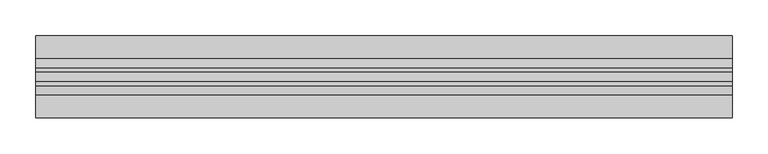
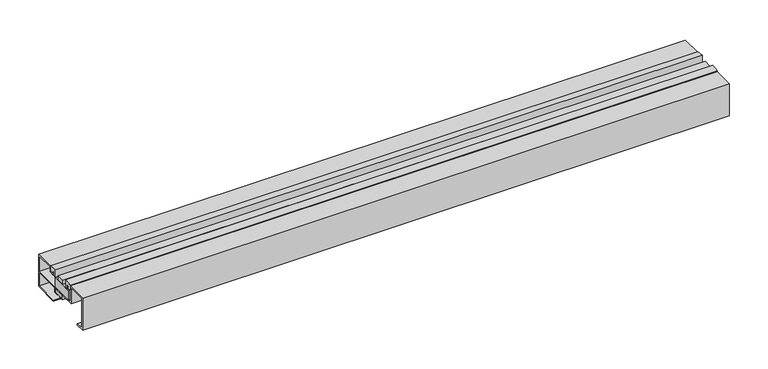
"""IFC4 building model written with IfcOpenShell, lengths in millimetres: proxy geometry, Generic Models 3:Generic Models 1:2:Generic Models 1:2 : Generic Models 3:Generic Models 1:300625:328150:Generic Models 1:2:Generic Models 1:2 : Generic Models 3:Generic Models 1:300625:328150 : Generic Models 3:Generic Models 1:2:Generic Models 1:2 : Generic Models 3:Generic Models 1:300625:328150:1 : Generic Models 3:Generic Models 1:2:Generic Models 1:2 : Generic Models 3:Generic Models 1:300625:328150:Generic Models 1:2:Generic Models 1:2 : Generic Models 3:Generic Models 1:300625:328150 : Generic Models 3:Generic Models 1:2:Generic Models 1:2 : Generic Models 3:Generic Models 1:300625:328150:300962."""

import ifcopenshell
import ifcopenshell.guid

model = None  # the IFC model being written
_history = None  # IfcOwnerHistory: only IFC2X3 demands one
_inside = {}  # id of a spatial element -> (the spatial element, [elements in it])
_under = {}  # id of a project, library or spatial element -> (it, [spatial elements below it])
_declared = {}  # id of a project -> (the project, [libraries it declares])
_typed = {}  # id of a type object -> (the type object, [elements of that type])
_made_of = {}  # id of a material, layer set ... -> (it, [elements and type objects made of it])


def new_model(schema):
    """Start an empty IFC model of exactly this schema.

    Asked for "IFC4X3", IfcOpenShell would pick the latest addendum, in which some entities
    have other attributes; the version numbers below select the first issue.
    IFC2X3 requires an IfcOwnerHistory on every rooted entity: one is made here for all.
    """
    global model, _history
    if schema == "IFC4X3":
        model = ifcopenshell.file(schema_version=(4, 3, 0, 0))
    else:
        model = ifcopenshell.file(schema=schema)
    _inside.clear()
    _under.clear()
    _declared.clear()
    _typed.clear()
    _made_of.clear()
    _history = None
    if model.schema == "IFC2X3":
        org = make("IfcOrganization", Name="unknown")
        user = make(
            "IfcPersonAndOrganization",
            ThePerson=make("IfcPerson", FamilyName="unknown"),
            TheOrganization=org,
        )
        app = make(
            "IfcApplication",
            ApplicationDeveloper=org,
            Version="unknown",
            ApplicationFullName="unknown",
            ApplicationIdentifier="unknown",
        )
        _history = make(
            "IfcOwnerHistory",
            OwningUser=user,
            OwningApplication=app,
            ChangeAction="ADDED",
            CreationDate=0,
        )
    return model


def make(cls, **values):
    """One entity of the class cls with the attributes given. An attribute that is None is left unset."""
    return model.create_entity(
        cls, **{name: value for name, value in values.items() if value is not None}
    )


def rooted(cls, **values):
    """An entity with a GlobalId (a new one), such as an element, a storey or a relation."""
    return make(cls, GlobalId=ifcopenshell.guid.new(), OwnerHistory=_history, **values)


def si_unit(unit_type, name, prefix=None):
    """IfcSIUnit, for example si_unit("LENGTHUNIT", "METRE", prefix="MILLI")."""
    return make("IfcSIUnit", UnitType=unit_type, Prefix=prefix, Name=name)


def assignment(units):
    """IfcUnitAssignment: the units of a project."""
    return None if units is None else make("IfcUnitAssignment", Units=units)


def point(xyz):
    """IfcCartesianPoint."""
    return None if xyz is None else make("IfcCartesianPoint", Coordinates=xyz)


def direction(xyz):
    """IfcDirection."""
    return None if xyz is None else make("IfcDirection", DirectionRatios=xyz)


def frame(location, z_axis=None, x_axis=None):
    """IfcAxis2Placement3D, a coordinate frame: its origin and axes. An axis left out is left unset."""
    return make(
        "IfcAxis2Placement3D",
        Location=point(location),
        Axis=direction(z_axis),
        RefDirection=direction(x_axis),
    )


def origin():
    """The frame at (0, 0, 0) with its axes left unset."""
    return frame((0.0, 0.0, 0.0))


def place(relative_to, where):
    """IfcLocalPlacement: puts the frame where relative to a parent placement (None: the world)."""
    return make(
        "IfcLocalPlacement", PlacementRelTo=relative_to, RelativePlacement=where
    )


def context(
    kind, dimensions, precision=None, world=None, true_north=None, identifier=None
):
    """IfcGeometricRepresentationContext, for example the 3D "Model" context."""
    return make(
        "IfcGeometricRepresentationContext",
        ContextIdentifier=identifier,
        ContextType=kind,
        CoordinateSpaceDimension=dimensions,
        Precision=precision,
        WorldCoordinateSystem=world,
        TrueNorth=true_north,
    )


def project(units=None, contexts=None):
    """IfcProject with its units and contexts."""
    return rooted(
        "IfcProject",
        Name="project",
        RepresentationContexts=contexts,
        UnitsInContext=assignment(units),
    )


def spatial(cls, under=None, at=None, **own):
    """A site, building, storey or space (cls), placed at a placement, below another one or the project."""
    s = rooted(cls, ObjectPlacement=at, **own)
    if under is not None:
        _under.setdefault(under.id(), (under, []))[1].append(s)
    return s


def polyline(points):
    """IfcPolyline through the points."""
    return make("IfcPolyline", Points=[point(p) for p in points])


def outline(outer, holes=None, kind="AREA"):
    """IfcArbitraryClosedProfileDef: a profile drawn as a closed curve; with holes, ...WithVoids."""
    if holes is None:
        return make("IfcArbitraryClosedProfileDef", ProfileType=kind, OuterCurve=outer)
    return make(
        "IfcArbitraryProfileDefWithVoids",
        ProfileType=kind,
        OuterCurve=outer,
        InnerCurves=holes,
    )


def extrude(swept, where, along, depth):
    """IfcExtrudedAreaSolid: the profile swept, set in the frame where, extruded along a direction by depth."""
    return make(
        "IfcExtrudedAreaSolid",
        SweptArea=swept,
        Position=where,
        ExtrudedDirection=direction(along),
        Depth=depth,
    )


def shape(context_of_items, identifier, shape_type, items):
    """IfcShapeRepresentation: the items that make up one representation, for example the "Body"."""
    return make(
        "IfcShapeRepresentation",
        ContextOfItems=context_of_items,
        RepresentationIdentifier=identifier,
        RepresentationType=shape_type,
        Items=items,
    )


def source(mapping_origin, context_of_items, identifier, shape_type, items):
    """IfcRepresentationMap: a shape defined once, which mapped items show again and again."""
    return make(
        "IfcRepresentationMap",
        MappingOrigin=mapping_origin,
        MappedRepresentation=shape(context_of_items, identifier, shape_type, items),
    )


def transform(
    local_origin,
    x_axis=None,
    y_axis=None,
    z_axis=None,
    scale=None,
    scale2=None,
    scale3=None,
    uniform=True,
):
    """IfcCartesianTransformationOperator3D, or its non-uniform kind. x_axis, y_axis, z_axis: its Axis1, 2, 3."""
    if uniform:
        return make(
            "IfcCartesianTransformationOperator3D",
            Axis1=direction(x_axis),
            Axis2=direction(y_axis),
            LocalOrigin=point(local_origin),
            Scale=scale,
            Axis3=direction(z_axis),
        )
    return make(
        "IfcCartesianTransformationOperator3DnonUniform",
        Axis1=direction(x_axis),
        Axis2=direction(y_axis),
        LocalOrigin=point(local_origin),
        Scale=scale,
        Axis3=direction(z_axis),
        Scale2=scale2,
        Scale3=scale3,
    )


def mapped(mapping_source, mapping_target):
    """IfcMappedItem: shows the shape of a source again, moved by a transform."""
    return make(
        "IfcMappedItem", MappingSource=mapping_source, MappingTarget=mapping_target
    )


def made_of(thing, what):
    """Note that an element or type object is made of a material, layer set ...; save() writes the relation."""
    if what is not None:
        _made_of.setdefault(what.id(), (what, []))[1].append(thing)
    return thing


def element(
    cls,
    number,
    at=None,
    inside=None,
    cuts=None,
    type_object=None,
    material=None,
    context=None,
    identifier="Body",
    shape_type=None,
    held_by="IfcProductDefinitionShape",
    body=None,
    shapes=None,
    **own,
):
    """One element of the class cls, such as IfcWall. Its Tag is "e" and its number.

    at: its placement. inside: the storey or other place that contains it. cuts: it is an
    opening in that element (IfcRelVoidsElement). A single representation is given by context,
    identifier, shape_type and body (its items); several are given by shapes. held_by: the class
    of the entity that holds the representations. save() writes the other relations.
    """
    e = rooted(cls, Tag="e%d" % number, ObjectPlacement=at, **own)
    if body is not None:
        shapes = [shape(context, identifier, shape_type, body)]
    if shapes is not None:
        e.Representation = make(held_by, Representations=shapes)
    if inside is not None:
        _inside.setdefault(inside.id(), (inside, []))[1].append(e)
    if cuts is not None:
        rooted(
            "IfcRelVoidsElement", RelatingBuildingElement=cuts, RelatedOpeningElement=e
        )
    if type_object is not None:
        _typed.setdefault(type_object.id(), (type_object, []))[1].append(e)
    return made_of(e, material)


def aggregate(whole, parts):
    """IfcRelAggregates: a whole, such as a stair, and the parts it consists of."""
    return rooted("IfcRelAggregates", RelatingObject=whole, RelatedObjects=parts)


def save(model, path):
    """Write the relations noted so far, then the file.

    IfcRelAggregates (storeys below a building ...), IfcRelContainedInSpatialStructure (elements
    in a storey), IfcRelDefinesByType, IfcRelAssociatesMaterial and IfcRelDeclares: one each for
    every whole, place, type object, material and project.
    """
    for whole, parts in _under.values():
        aggregate(whole, parts)
    for where, things in _inside.values():
        rooted(
            "IfcRelContainedInSpatialStructure",
            RelatedElements=things,
            RelatingStructure=where,
        )
    for kind, things in _typed.values():
        rooted("IfcRelDefinesByType", RelatedObjects=things, RelatingType=kind)
    for what, things in _made_of.values():
        rooted("IfcRelAssociatesMaterial", RelatedObjects=things, RelatingMaterial=what)
    for by, libraries in _declared.values():
        rooted("IfcRelDeclares", RelatingContext=by, RelatedDefinitions=libraries)
    model.write(path)


def generic_models_d3444f50(model_context):
    return source(origin(), model_context, "Body", "SweptSolid", [
        extrude(outline(polyline([(593731.7367239, -579047.2017564), (593731.7367239, -579080.4885915), (592761.7742239, -579080.4885915), (592761.7742239, -579047.2017564), (593731.7367239, -579047.2017564)])), frame((0.0, 0.0, 40.9290939), z_axis=(0.0, 0.0, 1.0), x_axis=(1.0, 0.0, 0.0)), (0.0, 0.0, 1.0), 14.2115027),
        extrude(outline(polyline([(593731.7367239, -579047.8857325), (593731.7367239, -579063.9971687), (592761.7742239, -579063.9971687), (592761.7742239, -579047.8857325), (593731.7367239, -579047.8857325)])), frame((0.0, 0.0, 32.9493731), z_axis=(0.0, 0.0, 1.0), x_axis=(1.0, 0.0, 0.0)), (0.0, 0.0, 1.0), 6.0797872),
        extrude(outline(polyline([(593731.7367239, -579054.6832724), (593731.7367239, -579067.3832724), (592761.7742239, -579067.3832724), (592761.7742239, -579054.6832724), (593731.7367239, -579054.6832724)])), frame((0.0, 0.0, 57.1165274), z_axis=(0.0, 0.0, 1.0), x_axis=(1.0, 0.0, 0.0)), (0.0, 0.0, 1.0), 6.3435484),
        extrude(outline(polyline([(-579078.8757591, 62.433193), (-579081.7214373, 62.433193), (-579081.7214373, 59.4893332), (-579086.0195091, 59.4893332), (-579086.0195091, 67.3290426), (-579074.1217032, 68.7899095), (-579074.1217032, 56.7196524), (-579078.8757591, 56.7196524), (-579078.8757591, 62.433193)])), frame((592761.7742239, 0.0, 0.0), z_axis=(1.0, 0.0, 0.0), x_axis=(0.0, 1.0, 0.0)), (0.0, 0.0, 1.0), 969.9625),
        extrude(outline(polyline([(-579036.0470357, 67.3290426), (-579036.0470357, 59.4893332), (-579040.3451075, 59.4893332), (-579040.3451075, 62.433193), (-579043.1907857, 62.433193), (-579043.1907857, 56.7196524), (-579047.9448415, 56.7196524), (-579047.9448415, 68.7899095), (-579036.0470357, 67.3290426)])), frame((592761.7742239, 0.0, 0.0), z_axis=(1.0, 0.0, 0.0), x_axis=(0.0, 1.0, 0.0)), (0.0, 0.0, 1.0), 969.9625),
        extrude(outline(polyline([(-579118.1663841, 15.5459822), (-579118.1663841, 66.3122056), (-579086.4163841, 66.3122056), (-579086.4163841, 59.0924582), (-579081.3245623, 59.0924582), (-579081.3245623, 62.036318), (-579079.2726341, 62.036318), (-579079.2726341, 57.1165274), (-579086.4163841, 57.1165274), (-579086.4163841, 40.9290939), (-579059.1333389, 40.9290939), (-579059.1333389, 39.0291604), (-579063.9971687, 39.0291604), (-579063.9971687, 32.9493731), (-579059.1333389, 32.9493731), (-579059.1333389, 31.6574183), (-579065.8971022, 31.6574183), (-579065.8971022, 39.0291604), (-579088.3163176, 39.0291604), (-579088.3163176, 64.4122721), (-579115.6584719, 64.4122721), (-579115.6584719, 17.4459157), (-579105.079253, 17.4459157), (-579105.079253, 15.5459822), (-579118.1663841, 15.5459822)])), frame((592761.7742239, 0.0, 0.0), z_axis=(1.0, 0.0, 0.0), x_axis=(0.0, 1.0, 0.0)), (0.0, 0.0, 1.0), 969.9625),
        extrude(outline(polyline([(-579040.7419825, 62.036318), (-579040.7419825, 59.0924582), (-579035.6501607, 59.0924582), (-579035.6501607, 66.3122056), (-579003.8663841, 66.3122056), (-579003.8663841, 15.5459822), (-579042.7939107, 15.5459822), (-579042.7939107, 17.4681948), (-579005.8423149, 17.4681948), (-579005.8423149, 39.0291604), (-579045.985799, 39.0291604), (-579045.985799, 31.6574183), (-579052.7495623, 31.6574183), (-579052.7495623, 32.9493731), (-579047.8857325, 32.9493731), (-579047.8857325, 39.0291604), (-579052.7495623, 39.0291604), (-579052.7495623, 40.9290939), (-579005.8423149, 40.9290939), (-579005.8423149, 64.4024065), (-579033.7502272, 64.4024065), (-579033.7502272, 57.1165274), (-579042.7939107, 57.1165274), (-579042.7939107, 62.036318), (-579040.7419825, 62.036318)])), frame((592761.7742239, 0.0, 0.0), z_axis=(1.0, 0.0, 0.0), x_axis=(0.0, 1.0, 0.0)), (0.0, 0.0, 1.0), 969.9625),
    ])


if __name__ == "__main__":
    model = new_model("IFC4")
    model_context = context("Model", 3, world=origin())
    ifc_project = project(units=[si_unit("LENGTHUNIT", "METRE", prefix="MILLI")], contexts=[model_context])
    site = spatial("IfcSite", under=ifc_project)
    building = spatial("IfcBuilding", under=site)
    placement = place(None, origin())
    generic_models_shape = generic_models_d3444f50(model_context)
    element("IfcBuildingElementProxy", 1, Name="Generic Models 3:Generic Models 1:2:Generic Models 1:2 : Generic Models 3:Generic Models 1:300625:328150:Generic Models 1:2:Generic Models 1:2 : Generic Models 3:Generic Models 1:300625:328150 : Generic Models 3:Generic Models 1:2:Generic Models 1:2 : Generic Models 3:Generic Models 1:300625:328150:1 : Generic Models 3:Generic Models 1:2:Generic Models 1:2 : Generic Models 3:Generic Models 1:300625:328150:Generic Models 1:2:Generic Models 1:2 : Generic Models 3:Generic Models 1:300625:328150 : Generic Models 3:Generic Models 1:2:Generic Models 1:2 : Generic Models 3:Generic Models 1:300625:328150:300962", ObjectType="Generic Models 3:Generic Models 1:2:Generic Models 1:2 : Generic Models 3:Generic Models 1:300625:328150:Generic Models 1:2:Generic Models 1:2 : Generic Models 3:Generic Models 1:300625:328150 : Generic Models 3:Generic Models 1:2:Generic Models 1:2 : Generic Models 3:Generic Models 1:300625:328150:1 : Generic Models 3:Generic Models 1:2:Generic Models 1:2 : Generic Models 3:Generic Models 1:300625:328150:Generic Models 1:2:Generic Models 1:2 : Generic Models 3:Generic Models 1:300625:328150 : Generic Models 3:Generic Models 1:2:Generic Models 1:2 : Generic Models 3:Generic Models 1:300625:328150:300962", at=placement, inside=building, context=model_context, shape_type="MappedRepresentation", body=[
        mapped(generic_models_shape, transform((0.0, 0.0, 0.0), x_axis=(1.0, 0.0, 0.0), y_axis=(0.0, 1.0, 0.0), z_axis=(0.0, 0.0, 1.0))),
    ])
    save(model, "model.ifc")

# Revit data of these elements
# Type "Generic Models 3:Generic Models 1:2:Generic Models 1:2 : Generic Models 3:Generic Models 1:300625:328150:Generic Models 1:2:Generic Models 1:2 : Generic Models 3:Generic Models 1:300625:328150 : Generic Models 3:Generic Models 1:2:Generic Models 1:2 : Generic Models 3:Generic Models 1:300625:328150:1 : Generic Models 3:Generic Models 1:2:Generic Models 1:2 : Generic Models 3:Generic Models 1:300625:328150:Generic Models 1:2:Generic Models 1:2 : Generic Models 3:Generic Models 1:300625:328150 : Generic Models 3:Generic Models 1:2:Generic Models 1:2 : Generic Models 3:Generic Models 1:300625:328150:300962"
#   NameOverride = "Generic Models 3:Generic Models 1:2:Generic Models 1:2 : Generic Models 3:Generic Models 1:300625:328150:Generic Models 1:2:Generic Models 1:2 : Generic Models 3:Generic Models 1:300625:328150 : Generic Models 3:Generic Models 1:2:Generic Models 1:2 : Generic Models 3:Generic Models 1:300625:328150:300962"
#   ObjectTypeOverride = "Generic Models 1:2:Generic Models 1:2 : Generic Models 3:Generic Models 1:300625:328150 : Generic Models 3:Generic Models 1:2:Generic Models 1:2 : Generic Models 3:Generic Models 1:300625:328150"
#   Reference = "Generic Models 1"
#   Tag = "300962"
# Element 1 (IfcBuildingElementProxy, "Generic Models 3:Generic Models 1:2:Generic Models 1:2 : Generic Models 3:Generic Models 1:300625:328150:Generic Models 1:2:Generic Models 1:2 : Generic Models 3:Generic Models 1:300625:328150 : Generic Models 3:Generic Models 1:2:Generic Models 1:2 : Generic Models 3:Generic Models 1:300625:328150:1 : Generic Models 3:Generic Models 1:2:Generic Models 1:2 : Generic Models 3:Generic Models 1:300625:328150:Generic Models 1:2:Generic Models 1:2 : Generic Models 3:Generic Models 1:300625:328150 : Generic Models 3:Generic Models 1:2:Generic Models 1:2 : Generic Models 3:Generic Models 1:300625:328150:300962")
#   Materials on its faces: "THERMAL BROKEN ALUMINUM STOREFRONT"
# Materials
#   "THERMAL BROKEN ALUMINUM STOREFRONT": class "Unassigned", colour RGB 244 244 244, transparency 0, Cost = 0
